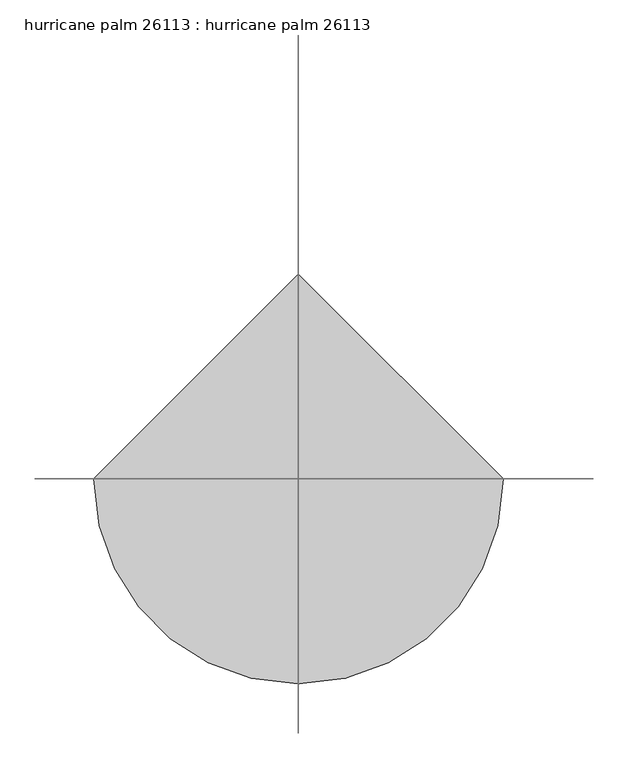
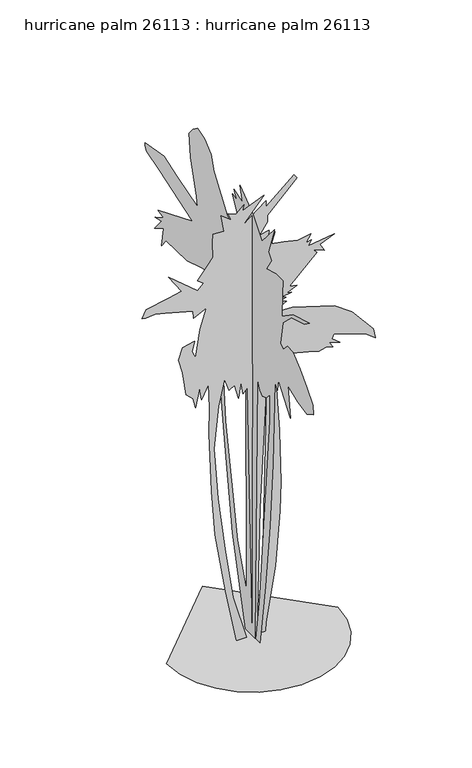
"""IFC4 building model written with IfcOpenShell, lengths in millimetres: proxy geometry, hurricane palm 26113 : hurricane palm 26113."""

from ifc_helpers import new_model, si_unit, origin, place, context, project, spatial, triangles, source, transform, mapped, element, save


def hurricane_palm_26113_hurricane_palm_26113_75f24be5(model_context):
    return source(origin(), model_context, "Body", "Tessellation", [
        triangles([(-654.0698874, 0.0, 0.0), (-636.7800997, -149.8698129, 0.0), (-587.5320883, -287.499875, 0.0), (-510.2755031, -408.9498928, 0.0), (-408.9498928, -510.2755031, 0.0), (-287.499875, -587.5320883, 0.0), (-149.8695585, -636.7800997, 0.0), (2.86e-05, -654.0698874, 0.0), (149.8698129, -636.7800997, 0.0), (287.499875, -587.5320883, 0.0), (408.9498928, -510.2755031, 0.0), (510.2755031, -408.9498928, 0.0), (587.5320883, -287.499875, 0.0), (636.7800997, -149.8695585, 0.0), (654.0698874, 5.72e-05, 0.0), (-8.58e-05, 654.0698874, 0.0), (318.8205832, -0.0001055, 3607.7882149), (342.0361719, -9.81e-05, 3572.9650497), (117.6189471, -7.01e-05, 3352.4168839), (117.6189471, -6.04e-05, 3298.2640846), (55.7107982, -4.76e-05, 3209.2625404), (129.2264781, -4.66e-05, 3224.731073), (125.3575554, -3.85e-05, 3178.2998955), (175.6579009, -3.94e-05, 3197.6548187), (148.5728899, -2.49e-05, 3108.6532745), (241.4349724, -1.74e-05, 3093.184742), (349.7755614, -7.1e-06, 3066.108197), (450.3747262, -5.5e-06, 3085.4375404), (411.6829382, 2.9e-06, 3027.3986412), (454.2431674, 3.7e-06, 3035.1455521), (431.0301221, 9.5e-06, 2996.4615761), (628.3600468, 1.46e-05, 3023.5378304), (516.1530876, 1.72e-05, 2977.1066528), (550.9764344, 3.01e-05, 2915.2069427), (465.8534689, 1.95e-05, 2950.0303986), (492.9374989, 2.64e-05, 2919.0677536), (283.9972182, 5.18e-05, 2717.874511), (342.0361719, 5.68e-05, 2706.2667892), (264.6500525, 5.85e-05, 2675.3041443), (299.4734356, 6.16e-05, 2667.5825226), (225.9582644, 6e-05, 2655.9748009), (256.9132246, 6.43e-05, 2640.4806885), (206.6115892, 6.45e-05, 2625.0121559), (260.7816294, 7.07e-05, 2605.6572327), (140.8345268, 7.5e-05, 2547.6183334), (307.2127888, 8.41e-05, 2543.7575226), (628.3600468, 0.0001184, 2443.1531982), (759.9166969, 0.0001423, 2346.42262), (926.2942595, 0.0001854, 2152.9585567), (941.7704224, 0.0002007, 2071.7039234), (875.9946407, 0.0001877, 2125.8744541), (624.4916056, 0.0001583, 2218.7368092), (609.0154063, 0.0001638, 2183.9134987), (670.9227831, 0.0001759, 2133.6113365), (589.6682588, 0.0001676, 2156.8269253), (616.7522524, 0.0001766, 2114.2667324), (562.5842288, 0.0001711, 2129.742968), (508.4136981, 0.0001704, 2118.1351009), (431.0301221, 0.0001631, 2137.4823212), (299.4734356, 0.0001502, 2172.3056316), (167.9192925, 0.0001345, 2222.605323), (206.6115892, 0.0002513, 1580.3081909), (218.219638, 0.0003259, 1166.2961071), (210.4810297, 0.0003671, 934.1402922), (179.5268326, 0.000443, 500.7835316), (106.0108984, 0.0005161, 71.2967382), (102.1417123, 0.0005293, 0.0040964), (55.7107982, 0.0005275, 6.75e-05), (86.664741, 0.0003795, 829.6726862), (117.6189471, 0.0001437, 2156.8269253), (59.5799798, 0.0003463, 1007.6579704), (36.3641412, 0.0005257, 0.0040988), (1.5408621, 0.0005239, 0.0041002), (-37.1515409, 0.0001615, 2013.6650242), (-71.9749172, 0.0001667, 1974.9731998), (-87.4518931, 0.0001479, 2075.5724373), (-102.9291188, 0.0001692, 1951.7576111), (-133.8833159, 0.0001469, 2067.8355549), (-176.4450439, 0.0001496, 2040.7489815), (-211.2684271, 0.0001299, 2141.3506897), (-257.700622, 0.0001635, 1940.1498894), (-292.5214617, 0.0002205, 1611.2632782), (-261.5690269, 0.0002961, 1197.2511217), (-207.3989867, 0.000375, 771.6337143), (-145.490856, 0.0004514, 361.4900353), (-44.8901515, 0.0005207, 0.0081326), (-118.4060902, 0.0005178, 0.0041047), (-203.5298188, 0.0004368, 427.2683604), (-284.7846156, 0.0003455, 914.7956881), (-311.8686092, 0.0002797, 1274.6371685), (-331.2157931, 0.000195, 1742.8173122), (-327.3448448, 0.0001579, 1951.7576111), (-335.084198, 0.0001229, 2145.2190582), (-385.3837804, 0.0001397, 2036.8806129), (-400.8625594, 0.000121, 2137.4823212), (-431.8175014, 0.0001457, 1990.4494354), (-451.1621418, 0.0001309, 2067.8355549), (-505.3326725, 0.0001191, 2118.1351009), (-532.4166661, 8.39e-05, 2307.7281796), (-563.3716444, 6.22e-05, 2419.9377548), (-532.4166661, 4.79e-05, 2508.9291252), (-439.5543474, 4.91e-05, 2528.2762001), (-458.901495, 6.2e-05, 2450.890226), (-431.8175014, 7.37e-05, 2392.8537975), (-396.9915748, 3.67e-05, 2609.5180435), (-350.5604336, 1.07e-05, 2768.1664993), (-447.2937006, 1.48e-05, 2717.874511), (-451.1621418, 4.2e-06, 2775.9134102), (-663.9708092, -1.69e-05, 2833.9523094), (-741.3569286, -2.43e-05, 2853.2816528), (-814.8721361, -2.66e-05, 2845.5603218), (-841.9586369, -2.94e-05, 2853.2816528), (-811.0036949, -3.82e-05, 2911.3208427), (-640.7552204, -3.58e-05, 2946.1440079), (-540.1560556, -3.49e-05, 2969.359742), (-640.7552204, -6.62e-05, 3116.4001854), (-416.3387587, -2.1e-05, 2926.8146645), (-373.775986, -2.71e-05, 2973.245842), (-416.3387587, -3.55e-05, 3008.0692978), (-342.8235875, -4.91e-05, 3104.7924637), (-300.260833, -5.66e-05, 3158.9705521), (-304.1317813, -7.76e-05, 3275.0486412), (-300.260833, -8.98e-05, 3344.6952621), (-215.1373588, -8.41e-05, 3336.9483513), (-238.3532019, -0.0001095, 3472.381073), (-160.9678273, -9.45e-05, 3410.4557831), (-184.1836704, -0.0001061, 3468.4946823), (-122.2752672, -9.81e-05, 3441.418428), (-64.2365587, -0.0001056, 3499.4573273), (-75.8440988, -9.78e-05, 3453.0261497), (90.5341814, -0.0001019, 3522.6730614), (-75.8440988, -7.64e-05, 3333.0875404), (106.0108984, -9.21e-05, 3472.381073), (106.0108984, -8.31e-05, 3422.0635048), (3.6e-06, 111.5414929, 2091.8410664), (2.7e-06, 138.6039035, 2014.5184605), (-9.1e-06, 181.1303321, 2238.7520119), (-1.55e-05, 212.059131, 2331.5355927), (-1.87e-05, 258.4524475, 2254.2156029), (-2.47e-05, 328.0408052, 2176.8928516), (-3.28e-05, 405.3634111, 2138.2341648), (-7.8e-06, 351.2385899, 1515.797303), (3.68e-05, 192.7289882, 653.6635168), (6.06e-05, 76.7468144, 317.3169322), (5e-06, 84.4790731, 2153.6976105), (-2.35e-05, 722.380616, 3657.5976746), (-1.2e-05, 633.4603895, 3626.6606094), (8e-07, 544.5400904, 3553.203756), (8.1e-06, 509.7471923, 3448.8351265), (2.39e-05, 413.0951703, 3305.7825211), (3.76e-05, 328.0408052, 3185.945359), (4.85e-05, 246.8535552, 3143.4002815), (5.72e-05, 157.9343097, 3209.1355133), (3.88e-05, 262.318327, 3406.3156288), (4.67e-05, 200.4607292, 3390.8470963), (3.98e-05, 242.9874212, 3452.6959373), (5.46e-05, 127.0055108, 3417.8980614), (4.69e-05, 161.799935, 3537.7605125), (7.16e-05, -12.1727138, 3406.3156288), (8.98e-05, -128.1548593, 3259.4022125), (0.0001038, -294.3959657, 3452.6959373), (0.0001008, -213.2082251, 3228.4648567), (0.0001074, -255.7346628, 3178.1984482), (0.0001022, -186.1458145, 3073.8298187), (0.0001164, -313.7253636, 3108.6276947), (0.0001274, -406.5114879, 3108.6276947), (0.0001299, -398.7797287, 2996.5121544), (0.0001348, -394.9138673, 2814.8008621), (0.0001489, -537.9589514, 2915.30839), (0.0001728, -754.4582365, 2977.1575218), (0.0001669, -692.6016924, 2930.7772133), (0.0001481, -522.4928896, 2880.5105141), (0.0001375, -406.5114879, 2772.2557846), (0.000139, -371.7160463, 2582.8228706), (0.0001443, -410.3773856, 2559.6324257), (0.000149, -464.5022069, 2617.6207466), (0.0001579, -537.9589514, 2613.7599358), (0.0001717, -634.6084299, 2536.4373299), (0.0001852, -723.5287291, 2439.787706), (0.0001976, -804.7172327, 2347.0016544), (0.0002007, -812.4489555, 2273.5449463), (0.0001916, -723.5287291, 2223.2859501), (0.0001765, -603.6814296, 2250.3497051), (0.0001597, -476.0998275, 2304.4744537), (0.0001703, -503.1635098, 2057.0456612), (0.0001455, -348.5208052, 2269.6790485), (0.0001463, -333.0572868, 2180.7613655), (0.0001413, -302.1277249, 2227.1518478), (0.0001582, -275.0640425, 1550.5902374), (0.0001693, -236.4045018, 1024.8055429), (0.0001778, -178.4135466, 506.752535), (0.0001841, -104.9583191, 0.0066211), (0.0001776, -50.8332435, 0.0066227), (0.0001732, -93.3601808, 321.1827936), (0.0001439, -236.4045018, 1875.3417812), (0.0001376, -236.4045018, 2087.9751686), (0.0001337, -190.011694, 2033.85042), (0.0001278, -135.8868637, 2014.5184605), (0.0001228, -101.0921852, 2041.5820702), (0.000117, -70.1636452, 2115.0363075), (0.0001762, -39.2348462, 0.0106537), (0.0001612, 88.3452071, 0.0066269), (0.0001208, 258.4524475, 672.9928602), (8.92e-05, 362.8362104, 1314.7616089), (5.46e-05, 463.3541302, 2072.5091068), (5.04e-05, 463.3541302, 2215.5541546), (4.58e-05, 513.6130537, 2169.1612015), (4.52e-05, 467.2199916, 2374.0627934), (3.97e-05, 509.7471923, 2389.5288551), (3.84e-05, 486.5493713, 2524.839782), (3.4e-05, 529.076572, 2501.6443954), (2.95e-05, 544.5400904, 2590.5697815), (1.56e-05, 668.2557947, 2563.4932365), (-5.6e-06, 861.5572952, 2501.6443954), (-3.86e-05, 1139.9157406, 2493.9125999), (-4.33e-05, 1197.9063869, 2420.4558918), (-4.46e-05, 1170.8427046, 2571.2404381), (-5.69e-05, 1290.6925838, 2505.5101479), (-4.92e-05, 1197.9063869, 2617.6207466), (-5.87e-05, 1282.9607883, 2598.2914032), (-4.77e-05, 1174.7111458, 2660.1402443), (-5.66e-05, 1244.2994854, 2679.4951675), (-8.2e-06, 791.9689556, 2865.0419815), (-6.51e-05, 1232.7017921, 3011.9553978), (-8.63e-05, 1398.9422264, 3058.3612862), (-8.96e-05, 1418.2715698, 3093.1591621), (-9.03e-05, 1418.2715698, 3116.3493164), (-6.16e-05, 1166.9768795, 3158.8691048), (-3.82e-05, 985.2729996, 3100.8807838), (-4.9e-06, 726.2465137, 3019.7025993), (-8.3e-06, 733.9782366, 3100.8807838), (-2.59e-05, 815.1667402, 3367.6313622), (-3.36e-05, 834.4961563, 3549.3429451), (-2.95e-05, 784.2372328, 3611.217366), (4.94e-05, 30.3542496, 2215.5541546), (0.0001139, 3.2915585, 158.8072942), (5.52e-05, -12.1726377, 2192.3589134)], [[15, 16, 1], [14, 15, 1], [14, 1, 2], [13, 14, 2], [13, 2, 3], [13, 3, 4], [12, 13, 4], [11, 12, 4], [11, 4, 5], [11, 5, 6], [11, 6, 7], [11, 7, 8], [11, 8, 9], [11, 9, 10], [31, 32, 33], [115, 116, 117], [39, 40, 41], [76, 77, 78], [53, 54, 55], [95, 96, 97], [130, 131, 132], [128, 129, 130], [37, 38, 39], [93, 94, 95], [33, 34, 35], [49, 50, 51], [31, 33, 35], [55, 56, 57], [124, 125, 126], [41, 42, 43], [126, 127, 128], [27, 28, 29], [43, 44, 45], [29, 30, 31], [74, 75, 76], [23, 24, 25], [132, 133, 134], [101, 102, 103], [106, 107, 108], [100, 101, 103], [21, 22, 23], [128, 130, 132], [126, 128, 132], [78, 79, 80], [85, 86, 87], [85, 87, 88], [84, 85, 88], [84, 88, 89], [83, 84, 89], [83, 89, 90], [82, 83, 90], [82, 90, 91], [81, 82, 91], [81, 91, 92], [48, 49, 51], [48, 51, 52], [111, 112, 113], [47, 48, 52], [110, 111, 113], [110, 113, 114], [109, 110, 114], [134, 17, 18], [134, 18, 19], [132, 134, 19], [95, 97, 98], [67, 68, 69], [66, 67, 69], [65, 66, 69], [64, 65, 69], [64, 69, 70], [63, 64, 70], [62, 63, 70], [61, 62, 70], [124, 126, 132], [132, 19, 20], [132, 20, 21], [95, 98, 99], [122, 123, 124], [99, 100, 103], [99, 103, 104], [72, 73, 74], [71, 72, 74], [70, 71, 74], [70, 74, 76], [118, 119, 120], [95, 99, 104], [93, 95, 104], [35, 36, 37], [80, 81, 92], [80, 92, 93], [108, 109, 114], [108, 114, 115], [108, 115, 117], [106, 108, 117], [31, 35, 37], [46, 47, 52], [46, 52, 53], [46, 53, 55], [46, 55, 57], [46, 57, 58], [46, 58, 59], [46, 59, 60], [46, 60, 61], [45, 46, 61], [80, 93, 104], [106, 117, 118], [29, 31, 37], [27, 29, 37], [26, 27, 37], [25, 26, 37], [121, 122, 124], [121, 124, 132], [121, 132, 21], [76, 78, 80], [80, 104, 105], [70, 76, 80], [70, 80, 105], [61, 70, 105], [45, 61, 105], [45, 105, 106], [43, 45, 106], [41, 43, 106], [41, 106, 118], [41, 118, 120], [41, 120, 121], [41, 121, 21], [41, 21, 23], [41, 23, 25], [41, 25, 37], [41, 37, 39], [235, 144, 145], [144, 235, 236], [219, 220, 221], [160, 161, 162], [169, 170, 171], [169, 171, 172], [217, 218, 219], [215, 216, 217], [184, 185, 186], [135, 136, 137], [168, 169, 172], [168, 172, 173], [206, 207, 208], [157, 158, 159], [221, 222, 223], [155, 156, 157], [186, 187, 188], [145, 135, 146], [145, 146, 147], [145, 147, 148], [145, 148, 149], [145, 149, 150], [145, 150, 151], [153, 154, 155], [145, 151, 152], [235, 145, 152], [210, 211, 212], [192, 193, 194], [191, 192, 194], [191, 194, 195], [190, 191, 195], [189, 190, 195], [188, 189, 195], [188, 195, 196], [165, 166, 167], [153, 155, 157], [153, 157, 159], [153, 159, 160], [226, 227, 228], [225, 226, 228], [224, 225, 228], [223, 224, 228], [223, 228, 229], [223, 229, 230], [208, 209, 210], [201, 202, 203], [162, 163, 164], [160, 162, 164], [153, 160, 164], [214, 215, 217], [164, 165, 167], [164, 167, 168], [235, 152, 153], [235, 153, 164], [235, 164, 168], [235, 168, 173], [235, 173, 174], [237, 235, 174], [237, 174, 175], [180, 181, 182], [179, 180, 182], [179, 182, 183], [179, 183, 184], [178, 179, 184], [177, 178, 184], [176, 177, 184], [175, 176, 184], [237, 175, 184], [237, 184, 186], [237, 186, 188], [237, 188, 196], [237, 196, 197], [217, 219, 221], [214, 217, 221], [214, 221, 223], [213, 214, 223], [212, 213, 223], [212, 223, 230], [197, 198, 199], [197, 199, 200], [237, 197, 200], [236, 237, 200], [236, 200, 201], [236, 201, 203], [144, 236, 203], [143, 144, 203], [142, 143, 203], [142, 203, 204], [142, 204, 205], [141, 142, 205], [141, 205, 206], [140, 141, 206], [140, 206, 208], [139, 140, 208], [138, 139, 208], [138, 208, 210], [232, 233, 234], [232, 234, 146], [231, 232, 146], [210, 212, 230], [138, 210, 230], [138, 230, 231], [138, 231, 146], [138, 146, 135], [138, 135, 137]], closed=False),
    ])


if __name__ == "__main__":
    model = new_model("IFC4")
    model_context = context("Model", 3, world=origin())
    ifc_project = project(units=[si_unit("LENGTHUNIT", "METRE", prefix="MILLI")], contexts=[model_context])
    site = spatial("IfcSite", under=ifc_project)
    building = spatial("IfcBuilding", under=site)
    placement = place(None, origin())
    hurricane_palm_26113_hurricane_palm_26113_shape = hurricane_palm_26113_hurricane_palm_26113_75f24be5(model_context)
    element("IfcBuildingElementProxy", 1, Name="hurricane palm 26113 : hurricane palm 26113", ObjectType="hurricane palm 26113 : hurricane palm 26113", at=placement, inside=building, context=model_context, shape_type="MappedRepresentation", body=[
        mapped(hurricane_palm_26113_hurricane_palm_26113_shape, transform((0.0, 0.0, 0.0), x_axis=(1.0, 0.0, 0.0), y_axis=(0.0, 1.0, 0.0), z_axis=(0.0, 0.0, 1.0))),
    ])
    save(model, "model.ifc")

# Revit data of these elements
# Type "hurricane palm 26113 : hurricane palm 26113"
#   built-in parameter 1005195 = "RPC-16-FXGL-UL7X-PH44-0000-ST1L-LVER-AU"
#   Height = 0
